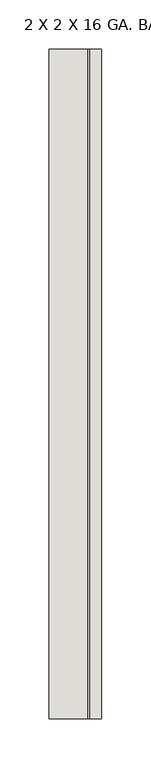
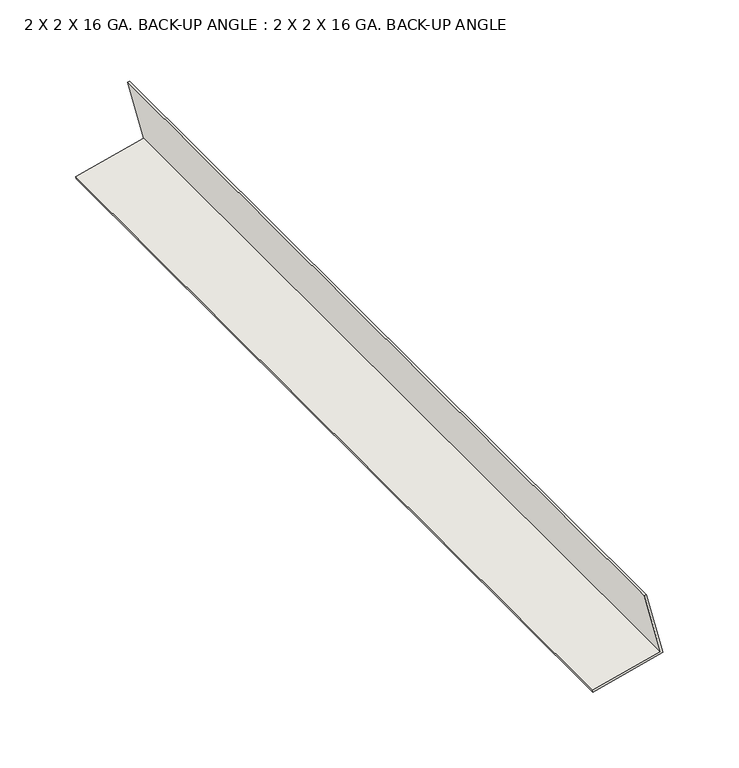
"""IFC4 building model written with IfcOpenShell, lengths in millimetres: wall geometry, 2 X 2 X 16 GA. BACK-UP ANGLE : 2 X 2 X 16 GA. BACK-UP ANGLE."""

from ifc_helpers import new_model, si_unit, frame, origin, place, context, project, spatial, polyline, outline, extrude, source, transform, mapped, element, save


def wall_2_x_2_x_16_ga_back_up_angle_2_x_2_x_16_ga_back_up_angle_1ad1ed1a(model_context):
    return source(origin(), model_context, "Body", "SweptSolid", [
        extrude(outline(polyline([(2933.991302, 19492.2682513), (2947.3787457, 19545.818026), (2998.202086, 19533.112191), (2997.8170607, 19531.5720898), (2948.5338216, 19543.8928995), (2935.5314033, 19491.883226), (2933.991302, 19492.2682513)])), frame((0.0, -2319.6634634, 0.0), z_axis=(0.0, 1.0, 0.0), x_axis=(0.0, 0.0, 1.0)), (0.0, 0.0, 1.0), 682.625),
    ])


if __name__ == "__main__":
    model = new_model("IFC4")
    model_context = context("Model", 3, world=origin())
    ifc_project = project(units=[si_unit("LENGTHUNIT", "METRE", prefix="MILLI")], contexts=[model_context])
    site = spatial("IfcSite", under=ifc_project)
    building = spatial("IfcBuilding", under=site)
    placement = place(None, origin())
    wall_2_x_2_x_16_ga_back_up_angle_2_x_2_x_16_ga_back_up_angle_shape = wall_2_x_2_x_16_ga_back_up_angle_2_x_2_x_16_ga_back_up_angle_1ad1ed1a(model_context)
    element("IfcWall", 1, ObjectType="2 X 2 X 16 GA. BACK-UP ANGLE : 2 X 2 X 16 GA. BACK-UP ANGLE", at=placement, inside=building, context=model_context, shape_type="MappedRepresentation", body=[
        mapped(wall_2_x_2_x_16_ga_back_up_angle_2_x_2_x_16_ga_back_up_angle_shape, transform((0.0, 0.0, 0.0), x_axis=(1.0, 0.0, 0.0), y_axis=(0.0, 1.0, 0.0), z_axis=(0.0, 0.0, 1.0))),
    ])
    save(model, "model.ifc")

# Revit data of these elements
# Element 1 (IfcWall, "2 X 2 X 16 GA. BACK-UP ANGLE : 2 X 2 X 16 GA. BACK-UP ANGLE")
#   Materials on its faces: "2 X 2 X 16 GA. BACK-UP ANGLE"
# Materials
#   "2 X 2 X 16 GA. BACK-UP ANGLE": class "Metal", colour RGB 247 247 247, transparency 0, Cost = 0
